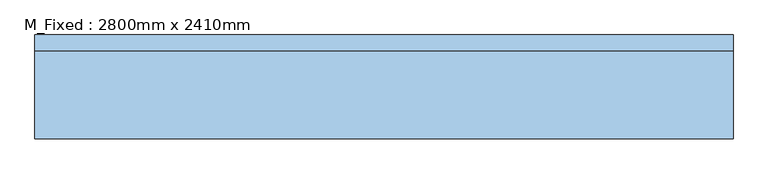
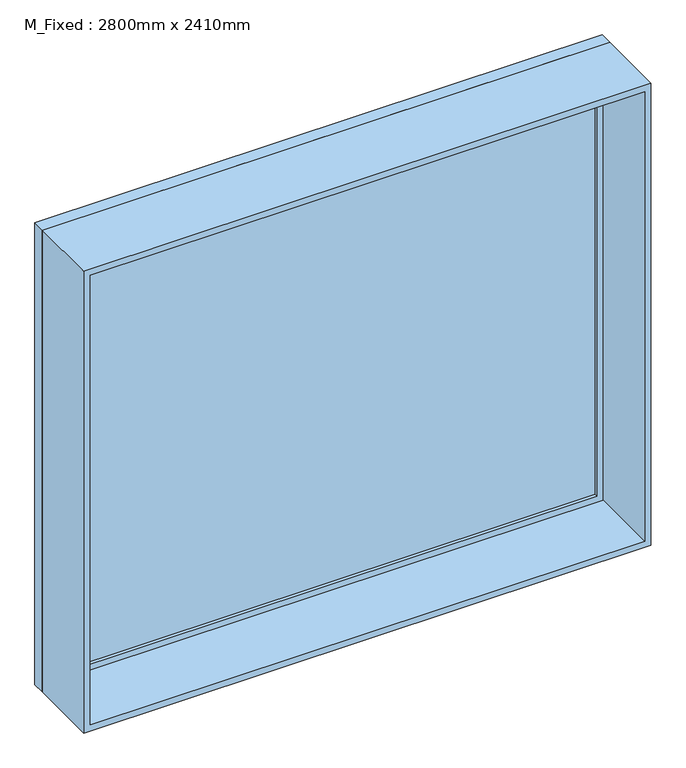
"""IFC4 building model written with IfcOpenShell, lengths in millimetres: window geometry, M_Fixed : 2800mm x 2410mm."""

import ifcopenshell
import ifcopenshell.guid

model = None  # the IFC model being written
_history = None  # IfcOwnerHistory: only IFC2X3 demands one
_inside = {}  # id of a spatial element -> (the spatial element, [elements in it])
_under = {}  # id of a project, library or spatial element -> (it, [spatial elements below it])
_declared = {}  # id of a project -> (the project, [libraries it declares])
_typed = {}  # id of a type object -> (the type object, [elements of that type])
_made_of = {}  # id of a material, layer set ... -> (it, [elements and type objects made of it])


def new_model(schema):
    """Start an empty IFC model of exactly this schema.

    Asked for "IFC4X3", IfcOpenShell would pick the latest addendum, in which some entities
    have other attributes; the version numbers below select the first issue.
    IFC2X3 requires an IfcOwnerHistory on every rooted entity: one is made here for all.
    """
    global model, _history
    if schema == "IFC4X3":
        model = ifcopenshell.file(schema_version=(4, 3, 0, 0))
    else:
        model = ifcopenshell.file(schema=schema)
    _inside.clear()
    _under.clear()
    _declared.clear()
    _typed.clear()
    _made_of.clear()
    _history = None
    if model.schema == "IFC2X3":
        org = make("IfcOrganization", Name="unknown")
        user = make(
            "IfcPersonAndOrganization",
            ThePerson=make("IfcPerson", FamilyName="unknown"),
            TheOrganization=org,
        )
        app = make(
            "IfcApplication",
            ApplicationDeveloper=org,
            Version="unknown",
            ApplicationFullName="unknown",
            ApplicationIdentifier="unknown",
        )
        _history = make(
            "IfcOwnerHistory",
            OwningUser=user,
            OwningApplication=app,
            ChangeAction="ADDED",
            CreationDate=0,
        )
    return model


def make(cls, **values):
    """One entity of the class cls with the attributes given. An attribute that is None is left unset."""
    return model.create_entity(
        cls, **{name: value for name, value in values.items() if value is not None}
    )


def rooted(cls, **values):
    """An entity with a GlobalId (a new one), such as an element, a storey or a relation."""
    return make(cls, GlobalId=ifcopenshell.guid.new(), OwnerHistory=_history, **values)


def si_unit(unit_type, name, prefix=None):
    """IfcSIUnit, for example si_unit("LENGTHUNIT", "METRE", prefix="MILLI")."""
    return make("IfcSIUnit", UnitType=unit_type, Prefix=prefix, Name=name)


def assignment(units):
    """IfcUnitAssignment: the units of a project."""
    return None if units is None else make("IfcUnitAssignment", Units=units)


def point(xyz):
    """IfcCartesianPoint."""
    return None if xyz is None else make("IfcCartesianPoint", Coordinates=xyz)


def direction(xyz):
    """IfcDirection."""
    return None if xyz is None else make("IfcDirection", DirectionRatios=xyz)


def frame(location, z_axis=None, x_axis=None):
    """IfcAxis2Placement3D, a coordinate frame: its origin and axes. An axis left out is left unset."""
    return make(
        "IfcAxis2Placement3D",
        Location=point(location),
        Axis=direction(z_axis),
        RefDirection=direction(x_axis),
    )


def origin():
    """The frame at (0, 0, 0) with its axes left unset."""
    return frame((0.0, 0.0, 0.0))


def place(relative_to, where):
    """IfcLocalPlacement: puts the frame where relative to a parent placement (None: the world)."""
    return make(
        "IfcLocalPlacement", PlacementRelTo=relative_to, RelativePlacement=where
    )


def context(
    kind, dimensions, precision=None, world=None, true_north=None, identifier=None
):
    """IfcGeometricRepresentationContext, for example the 3D "Model" context."""
    return make(
        "IfcGeometricRepresentationContext",
        ContextIdentifier=identifier,
        ContextType=kind,
        CoordinateSpaceDimension=dimensions,
        Precision=precision,
        WorldCoordinateSystem=world,
        TrueNorth=true_north,
    )


def project(units=None, contexts=None):
    """IfcProject with its units and contexts."""
    return rooted(
        "IfcProject",
        Name="project",
        RepresentationContexts=contexts,
        UnitsInContext=assignment(units),
    )


def spatial(cls, under=None, at=None, **own):
    """A site, building, storey or space (cls), placed at a placement, below another one or the project."""
    s = rooted(cls, ObjectPlacement=at, **own)
    if under is not None:
        _under.setdefault(under.id(), (under, []))[1].append(s)
    return s


def polyline(points):
    """IfcPolyline through the points."""
    return make("IfcPolyline", Points=[point(p) for p in points])


def outline(outer, holes=None, kind="AREA"):
    """IfcArbitraryClosedProfileDef: a profile drawn as a closed curve; with holes, ...WithVoids."""
    if holes is None:
        return make("IfcArbitraryClosedProfileDef", ProfileType=kind, OuterCurve=outer)
    return make(
        "IfcArbitraryProfileDefWithVoids",
        ProfileType=kind,
        OuterCurve=outer,
        InnerCurves=holes,
    )


def extrude(swept, where, along, depth):
    """IfcExtrudedAreaSolid: the profile swept, set in the frame where, extruded along a direction by depth."""
    return make(
        "IfcExtrudedAreaSolid",
        SweptArea=swept,
        Position=where,
        ExtrudedDirection=direction(along),
        Depth=depth,
    )


def shape(context_of_items, identifier, shape_type, items):
    """IfcShapeRepresentation: the items that make up one representation, for example the "Body"."""
    return make(
        "IfcShapeRepresentation",
        ContextOfItems=context_of_items,
        RepresentationIdentifier=identifier,
        RepresentationType=shape_type,
        Items=items,
    )


def source(mapping_origin, context_of_items, identifier, shape_type, items):
    """IfcRepresentationMap: a shape defined once, which mapped items show again and again."""
    return make(
        "IfcRepresentationMap",
        MappingOrigin=mapping_origin,
        MappedRepresentation=shape(context_of_items, identifier, shape_type, items),
    )


def transform(
    local_origin,
    x_axis=None,
    y_axis=None,
    z_axis=None,
    scale=None,
    scale2=None,
    scale3=None,
    uniform=True,
):
    """IfcCartesianTransformationOperator3D, or its non-uniform kind. x_axis, y_axis, z_axis: its Axis1, 2, 3."""
    if uniform:
        return make(
            "IfcCartesianTransformationOperator3D",
            Axis1=direction(x_axis),
            Axis2=direction(y_axis),
            LocalOrigin=point(local_origin),
            Scale=scale,
            Axis3=direction(z_axis),
        )
    return make(
        "IfcCartesianTransformationOperator3DnonUniform",
        Axis1=direction(x_axis),
        Axis2=direction(y_axis),
        LocalOrigin=point(local_origin),
        Scale=scale,
        Axis3=direction(z_axis),
        Scale2=scale2,
        Scale3=scale3,
    )


def mapped(mapping_source, mapping_target):
    """IfcMappedItem: shows the shape of a source again, moved by a transform."""
    return make(
        "IfcMappedItem", MappingSource=mapping_source, MappingTarget=mapping_target
    )


def made_of(thing, what):
    """Note that an element or type object is made of a material, layer set ...; save() writes the relation."""
    if what is not None:
        _made_of.setdefault(what.id(), (what, []))[1].append(thing)
    return thing


def element(
    cls,
    number,
    at=None,
    inside=None,
    cuts=None,
    type_object=None,
    material=None,
    context=None,
    identifier="Body",
    shape_type=None,
    held_by="IfcProductDefinitionShape",
    body=None,
    shapes=None,
    **own,
):
    """One element of the class cls, such as IfcWall. Its Tag is "e" and its number.

    at: its placement. inside: the storey or other place that contains it. cuts: it is an
    opening in that element (IfcRelVoidsElement). A single representation is given by context,
    identifier, shape_type and body (its items); several are given by shapes. held_by: the class
    of the entity that holds the representations. save() writes the other relations.
    """
    e = rooted(cls, Tag="e%d" % number, ObjectPlacement=at, **own)
    if body is not None:
        shapes = [shape(context, identifier, shape_type, body)]
    if shapes is not None:
        e.Representation = make(held_by, Representations=shapes)
    if inside is not None:
        _inside.setdefault(inside.id(), (inside, []))[1].append(e)
    if cuts is not None:
        rooted(
            "IfcRelVoidsElement", RelatingBuildingElement=cuts, RelatedOpeningElement=e
        )
    if type_object is not None:
        _typed.setdefault(type_object.id(), (type_object, []))[1].append(e)
    return made_of(e, material)


def aggregate(whole, parts):
    """IfcRelAggregates: a whole, such as a stair, and the parts it consists of."""
    return rooted("IfcRelAggregates", RelatingObject=whole, RelatedObjects=parts)


def save(model, path):
    """Write the relations noted so far, then the file.

    IfcRelAggregates (storeys below a building ...), IfcRelContainedInSpatialStructure (elements
    in a storey), IfcRelDefinesByType, IfcRelAssociatesMaterial and IfcRelDeclares: one each for
    every whole, place, type object, material and project.
    """
    for whole, parts in _under.values():
        aggregate(whole, parts)
    for where, things in _inside.values():
        rooted(
            "IfcRelContainedInSpatialStructure",
            RelatedElements=things,
            RelatingStructure=where,
        )
    for kind, things in _typed.values():
        rooted("IfcRelDefinesByType", RelatedObjects=things, RelatingType=kind)
    for what, things in _made_of.values():
        rooted("IfcRelAssociatesMaterial", RelatedObjects=things, RelatingMaterial=what)
    for by, libraries in _declared.values():
        rooted("IfcRelDeclares", RelatingContext=by, RelatedDefinitions=libraries)
    model.write(path)


def m_fixed_2800mm_x_2410mm_0fa4d817(model_context):
    return source(origin(), model_context, "Body", "SweptSolid", [
        extrude(outline(polyline([(-1337.0, 186.5), (1337.0, 186.5), (1337.0, 174.5), (-1337.0, 174.5), (-1337.0, 186.5)])), frame((0.0, 0.0, 163.0), z_axis=(0.0, 0.0, 1.0), x_axis=(1.0, 0.0, 0.0)), (0.0, 0.0, 1.0), 2284.0),
        extrude(outline(polyline([(2491.0, -1381.0), (119.0, -1381.0), (119.0, 1381.0), (2491.0, 1381.0), (2491.0, -1381.0)]), holes=[polyline([(2447.0, -1337.0), (2447.0, 1337.0), (163.0, 1337.0), (163.0, -1337.0), (2447.0, -1337.0)])]), frame((0.0, 158.5, 0.0), z_axis=(0.0, 1.0, 0.0), x_axis=(0.0, 0.0, 1.0)), (0.0, 0.0, 1.0), 44.0),
        extrude(outline(polyline([(2510.0, -1400.0), (100.0, -1400.0), (100.0, 1400.0), (2510.0, 1400.0), (2510.0, -1400.0)]), holes=[polyline([(2491.0, -1381.0), (2491.0, 1381.0), (119.0, 1381.0), (119.0, -1381.0), (2491.0, -1381.0)])]), frame((0.0, 158.5, 0.0), z_axis=(0.0, 1.0, 0.0), x_axis=(0.0, 0.0, 1.0)), (0.0, 0.0, 1.0), 63.0),
        extrude(outline(polyline([(2510.0, -1400.0), (100.0, -1400.0), (100.0, 1400.0), (2510.0, 1400.0), (2510.0, -1400.0)]), holes=[polyline([(2478.0, -1368.0), (2478.0, 1368.0), (132.0, 1368.0), (132.0, -1368.0), (2478.0, -1368.0)])]), frame((0.0, -195.5, 0.0), z_axis=(0.0, 1.0, 0.0), x_axis=(0.0, 0.0, 1.0)), (0.0, 0.0, 1.0), 354.0),
    ])


if __name__ == "__main__":
    model = new_model("IFC4")
    model_context = context("Model", 3, world=origin())
    ifc_project = project(units=[si_unit("LENGTHUNIT", "METRE", prefix="MILLI")], contexts=[model_context])
    site = spatial("IfcSite", under=ifc_project)
    building = spatial("IfcBuilding", under=site)
    placement = place(None, origin())
    m_fixed_2800mm_x_2410mm_shape = m_fixed_2800mm_x_2410mm_0fa4d817(model_context)
    element("IfcWindow", 1, ObjectType="M_Fixed : 2800mm x 2410mm", at=placement, inside=building, context=model_context, shape_type="MappedRepresentation", body=[
        mapped(m_fixed_2800mm_x_2410mm_shape, transform((0.0, 0.0, 0.0), x_axis=(1.0, 0.0, 0.0), y_axis=(0.0, 1.0, 0.0), z_axis=(0.0, 0.0, 1.0))),
    ])
    save(model, "model.ifc")

# Revit data of these elements
# Type "M_Fixed : 2800mm x 2410mm"
#   Manufacturer = "Manufacturer"
#   Type Mark = "01"
#   Construction Type = "Construction Type"
#   AccessibilityPerformance = "AccessibilityPerformance"
#   CodePerformance = "CodePerformance"
#   ConfigurationType = "ConfigurationType"
#   ConstructionType = "ConstructionType"
#   FireRating = "FireRating"
#   GlazingAreaFraction = "GlazingAreaFraction"
#   OperationType = "OperationType"
#   Area = "Area"
#   Color = "Color"
#   Constituents = "Constituents"
#   Features = "Features"
#   Finish = "Finish"
#   Grade = "Grade"
#   Material = "Material"
#   ModelReference = "ModelReference"
#   NominalHeight = "NominalHeight"
#   NominalLength = "NominalLength"
#   NominalWidth = "NominalWidth"
#   ProductionYear = "ProductionYear"
#   Reference = "Reference"
#   Shape = "Shape"
#   Size = "Size"
#   SustainabilityPerformance = "SustainabilityPerformance"
#   WarrantyDescription = "WarrantyDescription"
#   WarrantyDurationLabor = "WarrantyDurationLabor"
#   WarrantyDurationParts = "WarrantyDurationParts"
#   WarrantyGuarantorLabor = "WarrantyGuarantorLabor"
#   WarrantyGuarantorParts = "WarrantyGuarantorParts"
#   ExpectedLife = "ExpectedLife"
#   ReplacementCost = "ReplacementCost"
#   AssetAccountingType = "FIXED"
#   ModelLabel = "ModelLabel"
#   Height = 2.410 m
#   Default Sill Height = 0.100 m
#   Width = 2.800 m
#   Window Inset = 0.019 m
#   Frame Exterior Material = Sash
#   Frame Interior Material = Sash
#   Glass Pane Material = Glass
#   Sash = Sash
#   Wall Closure = (empty or 0)
# Element 1 (IfcWindow, "M_Fixed : 2800mm x 2410mm")
#   Materials on its faces: "Sash", "Glass"
# Materials
#   "Sash": class "Wood", colour RGB 224 178 126, transparency 0
#   "Glass": class "Glass", colour RGB 0 128 192, transparency 0.9
